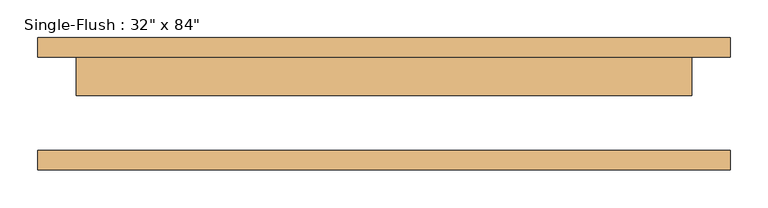
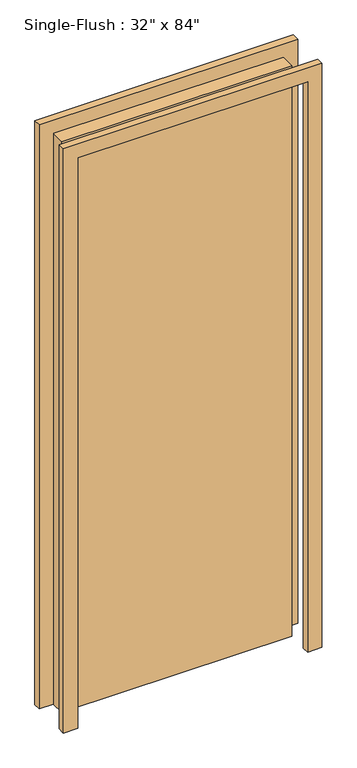
"""IFC4 building model written with IfcOpenShell, lengths in millimetres: door geometry."""

from ifc_helpers import new_model, si_unit, frame, origin, origin_with_axes, place, context, project, spatial, polyline, outline, extrude, source, transform, mapped, element, save


def door_4939ae0e(model_context):
    return source(origin(), model_context, "Body", "SweptSolid", [
        extrude(outline(polyline([(2184.4, -457.2), (0.0, -457.2), (0.0, -406.4), (2133.6, -406.4), (2133.6, 406.4), (0.0, 406.4), (0.0, 457.2), (2184.4, 457.2), (2184.4, -457.2)])), frame((0.0, 61.9125, 0.0), z_axis=(0.0, 1.0, 0.0), x_axis=(0.0, 0.0, 1.0)), (0.0, 0.0, 1.0), 25.4),
        extrude(outline(polyline([(2184.4, 457.2), (2184.4, -457.2), (0.0, -457.2), (0.0, -406.4), (2133.6, -406.4), (2133.6, 406.4), (0.0, 406.4), (0.0, 457.2), (2184.4, 457.2)])), frame((0.0, -87.3125, 0.0), z_axis=(0.0, 1.0, 0.0), x_axis=(0.0, 0.0, 1.0)), (0.0, 0.0, 1.0), 25.4),
        extrude(outline(polyline([(406.4, 11.1125), (-406.4, 11.1125), (-406.4, 61.9125), (406.4, 61.9125), (406.4, 11.1125)])), origin_with_axes(), (0.0, 0.0, 1.0), 2133.6),
    ])


if __name__ == "__main__":
    model = new_model("IFC4")
    model_context = context("Model", 3, world=origin())
    ifc_project = project(units=[si_unit("LENGTHUNIT", "METRE", prefix="MILLI")], contexts=[model_context])
    site = spatial("IfcSite", under=ifc_project)
    building = spatial("IfcBuilding", under=site)
    placement = place(None, origin())
    door_shape = door_4939ae0e(model_context)
    element("IfcDoor", 1, ObjectType="Single-Flush : 32\" x 84\"", at=placement, inside=building, context=model_context, shape_type="MappedRepresentation", body=[
        mapped(door_shape, transform((0.0, 0.0, 0.0), x_axis=(1.0, 0.0, 0.0), y_axis=(0.0, 1.0, 0.0), z_axis=(0.0, 0.0, 1.0))),
    ])
    save(model, "model.ifc")

# Revit data of these elements
# Type "Single-Flush : 32\" x 84\""
#   Type Mark = "10"
#   Construction Type Id = "MDOOR"
#   Assembly Code = "C1020"
#   Analytic Construction = "Metal"
#   Thickness = 0' - 2"
#   Heat Transfer Coefficient (U) = 3.7021 W/(m²·K)
#   Height = 7' - 0"
#   Trim Projection Ext = 0' - 1"
#   Trim Projection Int = 0' - 1"
#   Trim Width = 0' - 2"
#   Width = 2' - 8"
#   Door Material = Door - Panel
#   Frame Material = Door - Frame
#   Visual Light Transmittance = 0
#   Solar Heat Gain Coefficient = 0
#   Function = (empty or 0)
#   Wall Closure = (empty or 0)
# Element 1 (IfcDoor, "Single-Flush : 32\" x 84\"")
#   Materials on its faces: "Door - Frame", "Door - Panel"
# Materials
#   "Door - Panel": class "Wood", colour RGB 212 179 113, transparency 0, Cost = 0
#   "Door - Frame": class "Miscellaneous", colour RGB 65 65 65, transparency 0, Cost = 0
